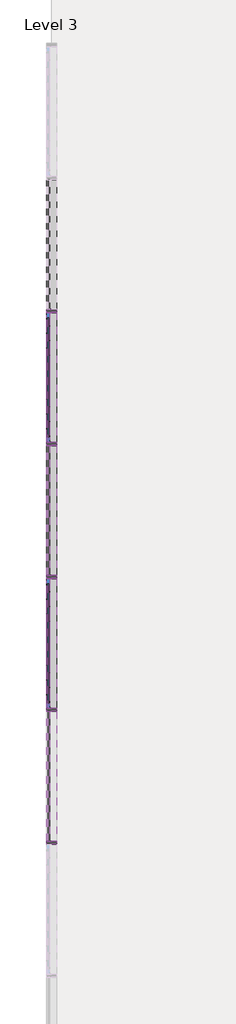
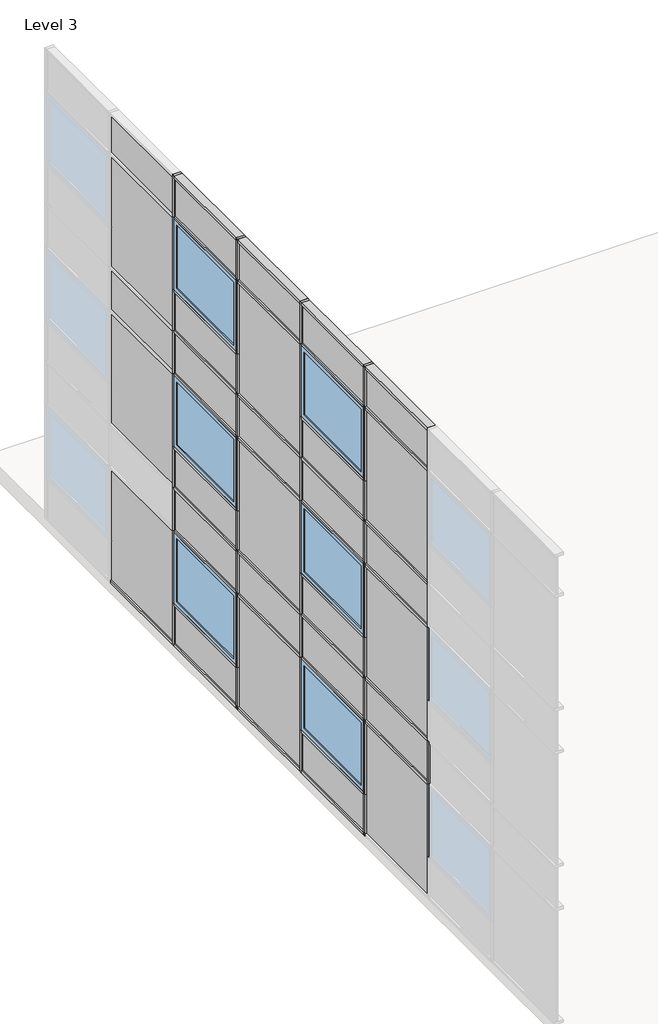
# One storey, part 4 of 5: 73 members, 29 plates, 6 windows.
"""IFC4 building model written with IfcOpenShell, lengths in millimetres."""

import ifcopenshell
import ifcopenshell.guid

model = None  # the IFC model being written
_history = None  # IfcOwnerHistory: only IFC2X3 demands one
_inside = {}  # id of a spatial element -> (the spatial element, [elements in it])
_under = {}  # id of a project, library or spatial element -> (it, [spatial elements below it])
_declared = {}  # id of a project -> (the project, [libraries it declares])
_typed = {}  # id of a type object -> (the type object, [elements of that type])
_made_of = {}  # id of a material, layer set ... -> (it, [elements and type objects made of it])


def new_model(schema):
    """Start an empty IFC model of exactly this schema.

    Asked for "IFC4X3", IfcOpenShell would pick the latest addendum, in which some entities
    have other attributes; the version numbers below select the first issue.
    IFC2X3 requires an IfcOwnerHistory on every rooted entity: one is made here for all.
    """
    global model, _history
    if schema == "IFC4X3":
        model = ifcopenshell.file(schema_version=(4, 3, 0, 0))
    else:
        model = ifcopenshell.file(schema=schema)
    _inside.clear()
    _under.clear()
    _declared.clear()
    _typed.clear()
    _made_of.clear()
    _history = None
    if model.schema == "IFC2X3":
        org = make("IfcOrganization", Name="unknown")
        user = make(
            "IfcPersonAndOrganization",
            ThePerson=make("IfcPerson", FamilyName="unknown"),
            TheOrganization=org,
        )
        app = make(
            "IfcApplication",
            ApplicationDeveloper=org,
            Version="unknown",
            ApplicationFullName="unknown",
            ApplicationIdentifier="unknown",
        )
        _history = make(
            "IfcOwnerHistory",
            OwningUser=user,
            OwningApplication=app,
            ChangeAction="ADDED",
            CreationDate=0,
        )
    return model


def make(cls, **values):
    """One entity of the class cls with the attributes given. An attribute that is None is left unset."""
    return model.create_entity(
        cls, **{name: value for name, value in values.items() if value is not None}
    )


def rooted(cls, **values):
    """An entity with a GlobalId (a new one), such as an element, a storey or a relation."""
    return make(cls, GlobalId=ifcopenshell.guid.new(), OwnerHistory=_history, **values)


def si_unit(unit_type, name, prefix=None):
    """IfcSIUnit, for example si_unit("LENGTHUNIT", "METRE", prefix="MILLI")."""
    return make("IfcSIUnit", UnitType=unit_type, Prefix=prefix, Name=name)


def assignment(units):
    """IfcUnitAssignment: the units of a project."""
    return None if units is None else make("IfcUnitAssignment", Units=units)


def point(xyz):
    """IfcCartesianPoint."""
    return None if xyz is None else make("IfcCartesianPoint", Coordinates=xyz)


def direction(xyz):
    """IfcDirection."""
    return None if xyz is None else make("IfcDirection", DirectionRatios=xyz)


def frame(location, z_axis=None, x_axis=None):
    """IfcAxis2Placement3D, a coordinate frame: its origin and axes. An axis left out is left unset."""
    return make(
        "IfcAxis2Placement3D",
        Location=point(location),
        Axis=direction(z_axis),
        RefDirection=direction(x_axis),
    )


def origin():
    """The frame at (0, 0, 0) with its axes left unset."""
    return frame((0.0, 0.0, 0.0))


def origin_with_axes():
    """The frame at (0, 0, 0) with the z axis (0, 0, 1) and the x axis (1, 0, 0) written out."""
    return frame((0.0, 0.0, 0.0), z_axis=(0.0, 0.0, 1.0), x_axis=(1.0, 0.0, 0.0))


def place(relative_to, where):
    """IfcLocalPlacement: puts the frame where relative to a parent placement (None: the world)."""
    return make(
        "IfcLocalPlacement", PlacementRelTo=relative_to, RelativePlacement=where
    )


def context(
    kind, dimensions, precision=None, world=None, true_north=None, identifier=None
):
    """IfcGeometricRepresentationContext, for example the 3D "Model" context."""
    return make(
        "IfcGeometricRepresentationContext",
        ContextIdentifier=identifier,
        ContextType=kind,
        CoordinateSpaceDimension=dimensions,
        Precision=precision,
        WorldCoordinateSystem=world,
        TrueNorth=true_north,
    )


def project(units=None, contexts=None):
    """IfcProject with its units and contexts."""
    return rooted(
        "IfcProject",
        Name="project",
        RepresentationContexts=contexts,
        UnitsInContext=assignment(units),
    )


def spatial(cls, under=None, at=None, **own):
    """A site, building, storey or space (cls), placed at a placement, below another one or the project."""
    s = rooted(cls, ObjectPlacement=at, **own)
    if under is not None:
        _under.setdefault(under.id(), (under, []))[1].append(s)
    return s


def polyline(points):
    """IfcPolyline through the points."""
    return make("IfcPolyline", Points=[point(p) for p in points])


def outline(outer, holes=None, kind="AREA"):
    """IfcArbitraryClosedProfileDef: a profile drawn as a closed curve; with holes, ...WithVoids."""
    if holes is None:
        return make("IfcArbitraryClosedProfileDef", ProfileType=kind, OuterCurve=outer)
    return make(
        "IfcArbitraryProfileDefWithVoids",
        ProfileType=kind,
        OuterCurve=outer,
        InnerCurves=holes,
    )


def extrude(swept, where, along, depth):
    """IfcExtrudedAreaSolid: the profile swept, set in the frame where, extruded along a direction by depth."""
    return make(
        "IfcExtrudedAreaSolid",
        SweptArea=swept,
        Position=where,
        ExtrudedDirection=direction(along),
        Depth=depth,
    )


def shape(context_of_items, identifier, shape_type, items):
    """IfcShapeRepresentation: the items that make up one representation, for example the "Body"."""
    return make(
        "IfcShapeRepresentation",
        ContextOfItems=context_of_items,
        RepresentationIdentifier=identifier,
        RepresentationType=shape_type,
        Items=items,
    )


def source(mapping_origin, context_of_items, identifier, shape_type, items):
    """IfcRepresentationMap: a shape defined once, which mapped items show again and again."""
    return make(
        "IfcRepresentationMap",
        MappingOrigin=mapping_origin,
        MappedRepresentation=shape(context_of_items, identifier, shape_type, items),
    )


def transform(
    local_origin,
    x_axis=None,
    y_axis=None,
    z_axis=None,
    scale=None,
    scale2=None,
    scale3=None,
    uniform=True,
):
    """IfcCartesianTransformationOperator3D, or its non-uniform kind. x_axis, y_axis, z_axis: its Axis1, 2, 3."""
    if uniform:
        return make(
            "IfcCartesianTransformationOperator3D",
            Axis1=direction(x_axis),
            Axis2=direction(y_axis),
            LocalOrigin=point(local_origin),
            Scale=scale,
            Axis3=direction(z_axis),
        )
    return make(
        "IfcCartesianTransformationOperator3DnonUniform",
        Axis1=direction(x_axis),
        Axis2=direction(y_axis),
        LocalOrigin=point(local_origin),
        Scale=scale,
        Axis3=direction(z_axis),
        Scale2=scale2,
        Scale3=scale3,
    )


def mapped(mapping_source, mapping_target):
    """IfcMappedItem: shows the shape of a source again, moved by a transform."""
    return make(
        "IfcMappedItem", MappingSource=mapping_source, MappingTarget=mapping_target
    )


def made_of(thing, what):
    """Note that an element or type object is made of a material, layer set ...; save() writes the relation."""
    if what is not None:
        _made_of.setdefault(what.id(), (what, []))[1].append(thing)
    return thing


def element(
    cls,
    number,
    at=None,
    inside=None,
    cuts=None,
    type_object=None,
    material=None,
    context=None,
    identifier="Body",
    shape_type=None,
    held_by="IfcProductDefinitionShape",
    body=None,
    shapes=None,
    **own,
):
    """One element of the class cls, such as IfcWall. Its Tag is "e" and its number.

    at: its placement. inside: the storey or other place that contains it. cuts: it is an
    opening in that element (IfcRelVoidsElement). A single representation is given by context,
    identifier, shape_type and body (its items); several are given by shapes. held_by: the class
    of the entity that holds the representations. save() writes the other relations.
    """
    e = rooted(cls, Tag="e%d" % number, ObjectPlacement=at, **own)
    if body is not None:
        shapes = [shape(context, identifier, shape_type, body)]
    if shapes is not None:
        e.Representation = make(held_by, Representations=shapes)
    if inside is not None:
        _inside.setdefault(inside.id(), (inside, []))[1].append(e)
    if cuts is not None:
        rooted(
            "IfcRelVoidsElement", RelatingBuildingElement=cuts, RelatedOpeningElement=e
        )
    if type_object is not None:
        _typed.setdefault(type_object.id(), (type_object, []))[1].append(e)
    return made_of(e, material)


def aggregate(whole, parts):
    """IfcRelAggregates: a whole, such as a stair, and the parts it consists of."""
    return rooted("IfcRelAggregates", RelatingObject=whole, RelatedObjects=parts)


def save(model, path):
    """Write the relations noted so far, then the file.

    IfcRelAggregates (storeys below a building ...), IfcRelContainedInSpatialStructure (elements
    in a storey), IfcRelDefinesByType, IfcRelAssociatesMaterial and IfcRelDeclares: one each for
    every whole, place, type object, material and project.
    """
    for whole, parts in _under.values():
        aggregate(whole, parts)
    for where, things in _inside.values():
        rooted(
            "IfcRelContainedInSpatialStructure",
            RelatedElements=things,
            RelatingStructure=where,
        )
    for kind, things in _typed.values():
        rooted("IfcRelDefinesByType", RelatedObjects=things, RelatingType=kind)
    for what, things in _made_of.values():
        rooted("IfcRelAssociatesMaterial", RelatedObjects=things, RelatingMaterial=what)
    for by, libraries in _declared.values():
        rooted("IfcRelDeclares", RelatingContext=by, RelatedDefinitions=libraries)
    model.write(path)


def rectangular_mullion_50_x_150mm_0967fd3c(model_context):
    return source(origin(), model_context, "Body", "SweptSolid", [
        extrude(outline(polyline([(0.0, 75.0), (0.0, -75.0), (-50.0, -75.0), (-50.0, 75.0), (0.0, 75.0)])), frame((0.0, 0.0, -1950.0000003), z_axis=(0.0, 0.0, 1.0), x_axis=(1.0, 0.0, 0.0)), (0.0, 0.0, 1.0), 1950.0000003),
    ])


def rectangular_mullion_50_x_150mm_f1645b81(model_context):
    return source(origin(), model_context, "Body", "SweptSolid", [
        extrude(outline(polyline([(25.0, 75.0), (25.0, -75.0), (-25.0, -75.0), (-25.0, 75.0), (25.0, 75.0)])), frame((0.0, 0.0, -1950.0000003), z_axis=(0.0, 0.0, 1.0), x_axis=(1.0, 0.0, 0.0)), (0.0, 0.0, 1.0), 1950.0000003),
    ])


def rectangular_mullion_50_x_150mm_14f10ac7(model_context):
    return source(origin(), model_context, "Body", "SweptSolid", [
        extrude(outline(polyline([(25.0, 75.0), (25.0, -75.0), (-25.0, -75.0), (-25.0, 75.0), (25.0, 75.0)])), frame((0.0, 0.0, -800.0), z_axis=(0.0, 0.0, 1.0), x_axis=(1.0, 0.0, 0.0)), (0.0, 0.0, 1.0), 800.0),
    ])


def rectangular_mullion_50_x_150mm_6270d9f9(model_context):
    return source(origin(), model_context, "Body", "SweptSolid", [
        extrude(outline(polyline([(25.0, 75.0), (25.0, -75.0), (-25.0, -75.0), (-25.0, 75.0), (25.0, 75.0)])), frame((0.0, 0.0, -775.0), z_axis=(0.0, 0.0, 1.0), x_axis=(1.0, 0.0, 0.0)), (0.0, 0.0, 1.0), 775.0),
    ])


def rectangular_mullion_50_x_150mm_80d7b263(model_context):
    return source(origin(), model_context, "Body", "SweptSolid", [
        extrude(outline(polyline([(25.0, 75.0), (25.0, -75.0), (-25.0, -75.0), (-25.0, 75.0), (25.0, 75.0)])), frame((0.0, 0.0, -1400.0), z_axis=(0.0, 0.0, 1.0), x_axis=(1.0, 0.0, 0.0)), (0.0, 0.0, 1.0), 1400.0),
    ])


def rectangular_mullion_50_x_150mm_9c26cac3(model_context):
    return source(origin(), model_context, "Body", "SweptSolid", [
        extrude(outline(polyline([(25.0, 75.0), (25.0, -75.0), (-25.0, -75.0), (-25.0, 75.0), (25.0, 75.0)])), frame((0.0, 0.0, -825.0), z_axis=(0.0, 0.0, 1.0), x_axis=(1.0, 0.0, 0.0)), (0.0, 0.0, 1.0), 825.0),
    ])


def system_panel_glazed_1e38db9b(model_context):
    return source(origin(), model_context, "Body", "SweptSolid", [
        extrude(outline(polyline([(0.0, -975.0000002), (0.0, 975.0000002), (750.0, 975.0000002), (2125.0, 975.0000002), (2125.0, -975.0000002), (750.0, -975.0000002), (0.0, -975.0000002)])), frame((0.0, 24.5, 0.0), z_axis=(0.0, 1.0, 0.0), x_axis=(0.0, 0.0, 1.0)), (0.0, 0.0, 1.0), 25.0),
    ])


def system_panel_glazed_bc1ebc0c(model_context):
    return source(origin(), model_context, "Body", "SweptSolid", [
        extrude(outline(polyline([(975.0000002, 24.5), (-975.0000002, 24.5), (-975.0000002, 49.5), (975.0000002, 49.5), (975.0000002, 24.5)])), origin_with_axes(), (0.0, 0.0, 1.0), 725.0),
    ])


def system_panel_glazed_d82c9dbb(model_context):
    return source(origin(), model_context, "Body", "SweptSolid", [
        extrude(outline(polyline([(975.0000002, 24.5), (-975.0000002, 24.5), (-975.0000002, 49.5), (975.0000002, 49.5), (975.0000002, 24.5)])), origin_with_axes(), (0.0, 0.0, 1.0), 775.0),
    ])


def m_curtain_wall_awning_m_curtain_wall_awning_db665c81(model_context):
    return source(origin(), model_context, "Body", "SweptSolid", [
        extrude(outline(polyline([(900.0, 44.05), (-900.0, 44.05), (-900.0, 56.75), (900.0, 56.75), (900.0, 44.05)])), frame((0.0, 0.0, 75.0), z_axis=(0.0, 0.0, 1.0), x_axis=(1.0, 0.0, 0.0)), (0.0, 0.0, 1.0), 1200.0),
        extrude(outline(polyline([(1350.0, -975.0), (0.0, -975.0), (0.0, 975.0), (1350.0, 975.0), (1350.0, -975.0)]), holes=[polyline([(1275.0, -900.0), (1275.0, 900.0), (75.0, 900.0), (75.0, -900.0), (1275.0, -900.0)])]), frame((0.0, 25.0, 0.0), z_axis=(0.0, 1.0, 0.0), x_axis=(0.0, 0.0, 1.0)), (0.0, 0.0, 1.0), 50.0),
    ])


model = new_model("IFC4")

# Units and contexts
model_context = context("Model", 3, world=origin())
ifc_project = project(units=[si_unit("LENGTHUNIT", "METRE", prefix="MILLI")], contexts=[model_context])

# Site, building, storey
site = spatial("IfcSite", under=ifc_project)
building = spatial("IfcBuilding", under=site)
storey = spatial("IfcBuildingStorey", under=building, Name="Level 3", Elevation=6000.0)

# Members
placement = place(None, origin())
rectangular_mullion_50_x_150mm_shape = rectangular_mullion_50_x_150mm_0967fd3c(model_context)
element("IfcMember", 1, ObjectType="Rectangular Mullion : 50 x 150mm", at=placement, inside=storey, context=model_context, shape_type="MappedRepresentation", body=[
    mapped(rectangular_mullion_50_x_150mm_shape, transform((-6732.0028633, 4048.7577233, 6000.0), x_axis=(0.0, 0.0, -1.0), y_axis=(1.0, 0.0, 0.0), z_axis=(0.0, -1.0, 0.0))),
])
element("IfcMember", 2, ObjectType="Rectangular Mullion : 50 x 150mm", at=placement, inside=storey, context=model_context, shape_type="MappedRepresentation", body=[
    mapped(rectangular_mullion_50_x_150mm_shape, transform((-6732.0028633, 6048.7577233, 6000.0), x_axis=(0.0, 0.0, -1.0), y_axis=(1.0, 0.0, 0.0), z_axis=(0.0, -1.0, 0.0))),
])
element("IfcMember", 3, ObjectType="Rectangular Mullion : 50 x 150mm", at=placement, inside=storey, context=model_context, shape_type="MappedRepresentation", body=[
    mapped(rectangular_mullion_50_x_150mm_shape, transform((-6732.0028633, 8048.7577233, 6000.0), x_axis=(0.0, 0.0, -1.0), y_axis=(1.0, 0.0, 0.0), z_axis=(0.0, -1.0, 0.0))),
])
element("IfcMember", 4, ObjectType="Rectangular Mullion : 50 x 150mm", at=placement, inside=storey, context=model_context, shape_type="MappedRepresentation", body=[
    mapped(rectangular_mullion_50_x_150mm_shape, transform((-6732.0028633, 10048.7577233, 6000.0), x_axis=(0.0, 0.0, -1.0), y_axis=(1.0, 0.0, 0.0), z_axis=(0.0, -1.0, 0.0))),
])
rectangular_mullion_50_x_150mm_2_shape = rectangular_mullion_50_x_150mm_f1645b81(model_context)
element("IfcMember", 5, ObjectType="Rectangular Mullion : 50 x 150mm", at=placement, inside=storey, context=model_context, shape_type="MappedRepresentation", body=[
    mapped(rectangular_mullion_50_x_150mm_2_shape, transform((-6732.0028633, 3998.7577233, 14200.0), x_axis=(0.0, 0.0, 1.0), y_axis=(1.0, 0.0, 0.0), z_axis=(0.0, 1.0, 0.0))),
])
element("IfcMember", 6, ObjectType="Rectangular Mullion : 50 x 150mm", at=placement, inside=storey, context=model_context, shape_type="MappedRepresentation", body=[
    mapped(rectangular_mullion_50_x_150mm_2_shape, transform((-6732.0028633, 5998.7577233, 14200.0), x_axis=(0.0, 0.0, 1.0), y_axis=(1.0, 0.0, 0.0), z_axis=(0.0, 1.0, 0.0))),
])
element("IfcMember", 7, ObjectType="Rectangular Mullion : 50 x 150mm", at=placement, inside=storey, context=model_context, shape_type="MappedRepresentation", body=[
    mapped(rectangular_mullion_50_x_150mm_2_shape, transform((-6732.0028633, 7998.7577233, 14200.0), x_axis=(0.0, 0.0, 1.0), y_axis=(1.0, 0.0, 0.0), z_axis=(0.0, 1.0, 0.0))),
])
element("IfcMember", 8, ObjectType="Rectangular Mullion : 50 x 150mm", at=placement, inside=storey, context=model_context, shape_type="MappedRepresentation", body=[
    mapped(rectangular_mullion_50_x_150mm_2_shape, transform((-6732.0028633, 9998.7577233, 14200.0), x_axis=(0.0, 0.0, 1.0), y_axis=(1.0, 0.0, 0.0), z_axis=(0.0, 1.0, 0.0))),
])
element("IfcMember", 9, ObjectType="Rectangular Mullion : 50 x 150mm", at=placement, inside=storey, context=model_context, shape_type="MappedRepresentation", body=[
    mapped(rectangular_mullion_50_x_150mm_2_shape, transform((-6732.0028633, 3998.7577233, 9025.0), x_axis=(0.0, 0.0, 1.0), y_axis=(1.0, 0.0, 0.0), z_axis=(0.0, 1.0, 0.0))),
])
element("IfcMember", 10, ObjectType="Rectangular Mullion : 50 x 150mm", at=placement, inside=storey, context=model_context, shape_type="MappedRepresentation", body=[
    mapped(rectangular_mullion_50_x_150mm_2_shape, transform((-6732.0028633, 5998.7577233, 9025.0), x_axis=(0.0, 0.0, 1.0), y_axis=(1.0, 0.0, 0.0), z_axis=(0.0, 1.0, 0.0))),
])
element("IfcMember", 11, ObjectType="Rectangular Mullion : 50 x 150mm", at=placement, inside=storey, context=model_context, shape_type="MappedRepresentation", body=[
    mapped(rectangular_mullion_50_x_150mm_2_shape, transform((-6732.0028633, 7998.7577233, 9025.0), x_axis=(0.0, 0.0, 1.0), y_axis=(1.0, 0.0, 0.0), z_axis=(0.0, 1.0, 0.0))),
])
element("IfcMember", 12, ObjectType="Rectangular Mullion : 50 x 150mm", at=placement, inside=storey, context=model_context, shape_type="MappedRepresentation", body=[
    mapped(rectangular_mullion_50_x_150mm_2_shape, transform((-6732.0028633, 9998.7577233, 9025.0), x_axis=(0.0, 0.0, 1.0), y_axis=(1.0, 0.0, 0.0), z_axis=(0.0, 1.0, 0.0))),
])
element("IfcMember", 13, ObjectType="Rectangular Mullion : 50 x 150mm", at=placement, inside=storey, context=model_context, shape_type="MappedRepresentation", body=[
    mapped(rectangular_mullion_50_x_150mm_2_shape, transform((-6732.0028633, 3998.7577233, 12025.0), x_axis=(0.0, 0.0, 1.0), y_axis=(1.0, 0.0, 0.0), z_axis=(0.0, 1.0, 0.0))),
])
element("IfcMember", 14, ObjectType="Rectangular Mullion : 50 x 150mm", at=placement, inside=storey, context=model_context, shape_type="MappedRepresentation", body=[
    mapped(rectangular_mullion_50_x_150mm_2_shape, transform((-6732.0028633, 5998.7577233, 12025.0), x_axis=(0.0, 0.0, 1.0), y_axis=(1.0, 0.0, 0.0), z_axis=(0.0, 1.0, 0.0))),
])
element("IfcMember", 15, ObjectType="Rectangular Mullion : 50 x 150mm", at=placement, inside=storey, context=model_context, shape_type="MappedRepresentation", body=[
    mapped(rectangular_mullion_50_x_150mm_2_shape, transform((-6732.0028633, 7998.7577233, 12025.0), x_axis=(0.0, 0.0, 1.0), y_axis=(1.0, 0.0, 0.0), z_axis=(0.0, 1.0, 0.0))),
])
element("IfcMember", 16, ObjectType="Rectangular Mullion : 50 x 150mm", at=placement, inside=storey, context=model_context, shape_type="MappedRepresentation", body=[
    mapped(rectangular_mullion_50_x_150mm_2_shape, transform((-6732.0028633, 9998.7577233, 12025.0), x_axis=(0.0, 0.0, 1.0), y_axis=(1.0, 0.0, 0.0), z_axis=(0.0, 1.0, 0.0))),
])
element("IfcMember", 17, ObjectType="Rectangular Mullion : 50 x 150mm", at=placement, inside=storey, context=model_context, shape_type="MappedRepresentation", body=[
    mapped(rectangular_mullion_50_x_150mm_2_shape, transform((-6732.0028633, 5998.7577233, 12800.0), x_axis=(0.0, 0.0, 1.0), y_axis=(1.0, 0.0, 0.0), z_axis=(0.0, 1.0, 0.0))),
])
element("IfcMember", 18, ObjectType="Rectangular Mullion : 50 x 150mm", at=placement, inside=storey, context=model_context, shape_type="MappedRepresentation", body=[
    mapped(rectangular_mullion_50_x_150mm_2_shape, transform((-6732.0028633, 9998.7577233, 12800.0), x_axis=(0.0, 0.0, 1.0), y_axis=(1.0, 0.0, 0.0), z_axis=(0.0, 1.0, 0.0))),
])
element("IfcMember", 19, ObjectType="Rectangular Mullion : 50 x 150mm", at=placement, inside=storey, context=model_context, shape_type="MappedRepresentation", body=[
    mapped(rectangular_mullion_50_x_150mm_2_shape, transform((-6732.0028633, 3998.7577233, 11200.0), x_axis=(0.0, 0.0, 1.0), y_axis=(1.0, 0.0, 0.0), z_axis=(0.0, 1.0, 0.0))),
])
element("IfcMember", 20, ObjectType="Rectangular Mullion : 50 x 150mm", at=placement, inside=storey, context=model_context, shape_type="MappedRepresentation", body=[
    mapped(rectangular_mullion_50_x_150mm_2_shape, transform((-6732.0028633, 5998.7577233, 11200.0), x_axis=(0.0, 0.0, 1.0), y_axis=(1.0, 0.0, 0.0), z_axis=(0.0, 1.0, 0.0))),
])
element("IfcMember", 21, ObjectType="Rectangular Mullion : 50 x 150mm", at=placement, inside=storey, context=model_context, shape_type="MappedRepresentation", body=[
    mapped(rectangular_mullion_50_x_150mm_2_shape, transform((-6732.0028633, 7998.7577233, 11200.0), x_axis=(0.0, 0.0, 1.0), y_axis=(1.0, 0.0, 0.0), z_axis=(0.0, 1.0, 0.0))),
])
element("IfcMember", 22, ObjectType="Rectangular Mullion : 50 x 150mm", at=placement, inside=storey, context=model_context, shape_type="MappedRepresentation", body=[
    mapped(rectangular_mullion_50_x_150mm_2_shape, transform((-6732.0028633, 9998.7577233, 11200.0), x_axis=(0.0, 0.0, 1.0), y_axis=(1.0, 0.0, 0.0), z_axis=(0.0, 1.0, 0.0))),
])
element("IfcMember", 23, ObjectType="Rectangular Mullion : 50 x 150mm", at=placement, inside=storey, context=model_context, shape_type="MappedRepresentation", body=[
    mapped(rectangular_mullion_50_x_150mm_2_shape, transform((-6732.0028633, 5998.7577233, 9800.0), x_axis=(0.0, 0.0, 1.0), y_axis=(1.0, 0.0, 0.0), z_axis=(0.0, 1.0, 0.0))),
])
element("IfcMember", 24, ObjectType="Rectangular Mullion : 50 x 150mm", at=placement, inside=storey, context=model_context, shape_type="MappedRepresentation", body=[
    mapped(rectangular_mullion_50_x_150mm_2_shape, transform((-6732.0028633, 9998.7577233, 9800.0), x_axis=(0.0, 0.0, 1.0), y_axis=(1.0, 0.0, 0.0), z_axis=(0.0, 1.0, 0.0))),
])
element("IfcMember", 25, ObjectType="Rectangular Mullion : 50 x 150mm", at=placement, inside=storey, context=model_context, shape_type="MappedRepresentation", body=[
    mapped(rectangular_mullion_50_x_150mm_2_shape, transform((-6732.0028633, 3998.7577233, 8200.0), x_axis=(0.0, 0.0, 1.0), y_axis=(1.0, 0.0, 0.0), z_axis=(0.0, 1.0, 0.0))),
])
element("IfcMember", 26, ObjectType="Rectangular Mullion : 50 x 150mm", at=placement, inside=storey, context=model_context, shape_type="MappedRepresentation", body=[
    mapped(rectangular_mullion_50_x_150mm_2_shape, transform((-6732.0028633, 5998.7577233, 8200.0), x_axis=(0.0, 0.0, 1.0), y_axis=(1.0, 0.0, 0.0), z_axis=(0.0, 1.0, 0.0))),
])
element("IfcMember", 27, ObjectType="Rectangular Mullion : 50 x 150mm", at=placement, inside=storey, context=model_context, shape_type="MappedRepresentation", body=[
    mapped(rectangular_mullion_50_x_150mm_2_shape, transform((-6732.0028633, 7998.7577233, 8200.0), x_axis=(0.0, 0.0, 1.0), y_axis=(1.0, 0.0, 0.0), z_axis=(0.0, 1.0, 0.0))),
])
element("IfcMember", 28, ObjectType="Rectangular Mullion : 50 x 150mm", at=placement, inside=storey, context=model_context, shape_type="MappedRepresentation", body=[
    mapped(rectangular_mullion_50_x_150mm_2_shape, transform((-6732.0028633, 9998.7577233, 8200.0), x_axis=(0.0, 0.0, 1.0), y_axis=(1.0, 0.0, 0.0), z_axis=(0.0, 1.0, 0.0))),
])
element("IfcMember", 29, ObjectType="Rectangular Mullion : 50 x 150mm", at=placement, inside=storey, context=model_context, shape_type="MappedRepresentation", body=[
    mapped(rectangular_mullion_50_x_150mm_2_shape, transform((-6732.0028633, 5998.7577233, 6800.0), x_axis=(0.0, 0.0, 1.0), y_axis=(1.0, 0.0, 0.0), z_axis=(0.0, 1.0, 0.0))),
])
element("IfcMember", 30, ObjectType="Rectangular Mullion : 50 x 150mm", at=placement, inside=storey, context=model_context, shape_type="MappedRepresentation", body=[
    mapped(rectangular_mullion_50_x_150mm_2_shape, transform((-6732.0028633, 9998.7577233, 6800.0), x_axis=(0.0, 0.0, 1.0), y_axis=(1.0, 0.0, 0.0), z_axis=(0.0, 1.0, 0.0))),
])
rectangular_mullion_50_x_150mm_3_shape = rectangular_mullion_50_x_150mm_14f10ac7(model_context)
element("IfcMember", 31, ObjectType="Rectangular Mullion : 50 x 150mm", at=placement, inside=storey, context=model_context, shape_type="MappedRepresentation", body=[
    mapped(rectangular_mullion_50_x_150mm_3_shape, transform((-6732.0028633, 4023.7577233, 6000.0), x_axis=(0.0, 1.0, 0.0), y_axis=(1.0, 0.0, 0.0), z_axis=(0.0, 0.0, -1.0))),
])
element("IfcMember", 32, ObjectType="Rectangular Mullion : 50 x 150mm", at=placement, inside=storey, context=model_context, shape_type="MappedRepresentation", body=[
    mapped(rectangular_mullion_50_x_150mm_3_shape, transform((-6732.0028633, 6023.7577233, 6000.0), x_axis=(0.0, 1.0, 0.0), y_axis=(1.0, 0.0, 0.0), z_axis=(0.0, 0.0, -1.0))),
])
element("IfcMember", 33, ObjectType="Rectangular Mullion : 50 x 150mm", at=placement, inside=storey, context=model_context, shape_type="MappedRepresentation", body=[
    mapped(rectangular_mullion_50_x_150mm_3_shape, transform((-6732.0028633, 8023.7577233, 6000.0), x_axis=(0.0, 1.0, 0.0), y_axis=(1.0, 0.0, 0.0), z_axis=(0.0, 0.0, -1.0))),
])
element("IfcMember", 34, ObjectType="Rectangular Mullion : 50 x 150mm", at=placement, inside=storey, context=model_context, shape_type="MappedRepresentation", body=[
    mapped(rectangular_mullion_50_x_150mm_3_shape, transform((-6732.0028633, 10023.7577233, 6000.0), x_axis=(0.0, 1.0, 0.0), y_axis=(1.0, 0.0, 0.0), z_axis=(0.0, 0.0, -1.0))),
])
element("IfcMember", 35, ObjectType="Rectangular Mullion : 50 x 150mm", at=placement, inside=storey, context=model_context, shape_type="MappedRepresentation", body=[
    mapped(rectangular_mullion_50_x_150mm_shape, transform((-6732.0028633, 3998.7577233, 15000.0), x_axis=(0.0, 0.0, 1.0), y_axis=(1.0, 0.0, 0.0), z_axis=(0.0, 1.0, 0.0))),
])
element("IfcMember", 36, ObjectType="Rectangular Mullion : 50 x 150mm", at=placement, inside=storey, context=model_context, shape_type="MappedRepresentation", body=[
    mapped(rectangular_mullion_50_x_150mm_shape, transform((-6732.0028633, 5998.7577233, 15000.0), x_axis=(0.0, 0.0, 1.0), y_axis=(1.0, 0.0, 0.0), z_axis=(0.0, 1.0, 0.0))),
])
element("IfcMember", 37, ObjectType="Rectangular Mullion : 50 x 150mm", at=placement, inside=storey, context=model_context, shape_type="MappedRepresentation", body=[
    mapped(rectangular_mullion_50_x_150mm_shape, transform((-6732.0028633, 7998.7577233, 15000.0), x_axis=(0.0, 0.0, 1.0), y_axis=(1.0, 0.0, 0.0), z_axis=(0.0, 1.0, 0.0))),
])
element("IfcMember", 38, ObjectType="Rectangular Mullion : 50 x 150mm", at=placement, inside=storey, context=model_context, shape_type="MappedRepresentation", body=[
    mapped(rectangular_mullion_50_x_150mm_shape, transform((-6732.0028633, 9998.7577233, 15000.0), x_axis=(0.0, 0.0, 1.0), y_axis=(1.0, 0.0, 0.0), z_axis=(0.0, 1.0, 0.0))),
])
element("IfcMember", 39, ObjectType="Rectangular Mullion : 50 x 150mm", at=placement, inside=storey, context=model_context, shape_type="MappedRepresentation", body=[
    mapped(rectangular_mullion_50_x_150mm_3_shape, transform((-6732.0028633, 4023.7577233, 14200.0), x_axis=(0.0, 1.0, 0.0), y_axis=(1.0, 0.0, 0.0), z_axis=(0.0, 0.0, -1.0))),
])
element("IfcMember", 40, ObjectType="Rectangular Mullion : 50 x 150mm", at=placement, inside=storey, context=model_context, shape_type="MappedRepresentation", body=[
    mapped(rectangular_mullion_50_x_150mm_3_shape, transform((-6732.0028633, 6023.7577233, 14200.0), x_axis=(0.0, 1.0, 0.0), y_axis=(1.0, 0.0, 0.0), z_axis=(0.0, 0.0, -1.0))),
])
element("IfcMember", 41, ObjectType="Rectangular Mullion : 50 x 150mm", at=placement, inside=storey, context=model_context, shape_type="MappedRepresentation", body=[
    mapped(rectangular_mullion_50_x_150mm_3_shape, transform((-6732.0028633, 8023.7577233, 14200.0), x_axis=(0.0, 1.0, 0.0), y_axis=(1.0, 0.0, 0.0), z_axis=(0.0, 0.0, -1.0))),
])
element("IfcMember", 42, ObjectType="Rectangular Mullion : 50 x 150mm", at=placement, inside=storey, context=model_context, shape_type="MappedRepresentation", body=[
    mapped(rectangular_mullion_50_x_150mm_3_shape, transform((-6732.0028633, 10023.7577233, 14200.0), x_axis=(0.0, 1.0, 0.0), y_axis=(1.0, 0.0, 0.0), z_axis=(0.0, 0.0, -1.0))),
])
rectangular_mullion_50_x_150mm_4_shape = rectangular_mullion_50_x_150mm_6270d9f9(model_context)
element("IfcMember", 43, ObjectType="Rectangular Mullion : 50 x 150mm", at=placement, inside=storey, context=model_context, shape_type="MappedRepresentation", body=[
    mapped(rectangular_mullion_50_x_150mm_4_shape, transform((-6732.0028633, 4023.7577233, 9025.0), x_axis=(0.0, 1.0, 0.0), y_axis=(1.0, 0.0, 0.0), z_axis=(0.0, 0.0, -1.0))),
])
element("IfcMember", 44, ObjectType="Rectangular Mullion : 50 x 150mm", at=placement, inside=storey, context=model_context, shape_type="MappedRepresentation", body=[
    mapped(rectangular_mullion_50_x_150mm_4_shape, transform((-6732.0028633, 4023.7577233, 12025.0), x_axis=(0.0, 1.0, 0.0), y_axis=(1.0, 0.0, 0.0), z_axis=(0.0, 0.0, -1.0))),
])
element("IfcMember", 45, ObjectType="Rectangular Mullion : 50 x 150mm", at=placement, inside=storey, context=model_context, shape_type="MappedRepresentation", body=[
    mapped(rectangular_mullion_50_x_150mm_4_shape, transform((-6732.0028633, 6023.7577233, 9025.0), x_axis=(0.0, 1.0, 0.0), y_axis=(1.0, 0.0, 0.0), z_axis=(0.0, 0.0, -1.0))),
])
element("IfcMember", 46, ObjectType="Rectangular Mullion : 50 x 150mm", at=placement, inside=storey, context=model_context, shape_type="MappedRepresentation", body=[
    mapped(rectangular_mullion_50_x_150mm_4_shape, transform((-6732.0028633, 6023.7577233, 12025.0), x_axis=(0.0, 1.0, 0.0), y_axis=(1.0, 0.0, 0.0), z_axis=(0.0, 0.0, -1.0))),
])
element("IfcMember", 47, ObjectType="Rectangular Mullion : 50 x 150mm", at=placement, inside=storey, context=model_context, shape_type="MappedRepresentation", body=[
    mapped(rectangular_mullion_50_x_150mm_4_shape, transform((-6732.0028633, 8023.7577233, 9025.0), x_axis=(0.0, 1.0, 0.0), y_axis=(1.0, 0.0, 0.0), z_axis=(0.0, 0.0, -1.0))),
])
element("IfcMember", 48, ObjectType="Rectangular Mullion : 50 x 150mm", at=placement, inside=storey, context=model_context, shape_type="MappedRepresentation", body=[
    mapped(rectangular_mullion_50_x_150mm_4_shape, transform((-6732.0028633, 8023.7577233, 12025.0), x_axis=(0.0, 1.0, 0.0), y_axis=(1.0, 0.0, 0.0), z_axis=(0.0, 0.0, -1.0))),
])
element("IfcMember", 49, ObjectType="Rectangular Mullion : 50 x 150mm", at=placement, inside=storey, context=model_context, shape_type="MappedRepresentation", body=[
    mapped(rectangular_mullion_50_x_150mm_4_shape, transform((-6732.0028633, 10023.7577233, 9025.0), x_axis=(0.0, 1.0, 0.0), y_axis=(1.0, 0.0, 0.0), z_axis=(0.0, 0.0, -1.0))),
])
element("IfcMember", 50, ObjectType="Rectangular Mullion : 50 x 150mm", at=placement, inside=storey, context=model_context, shape_type="MappedRepresentation", body=[
    mapped(rectangular_mullion_50_x_150mm_4_shape, transform((-6732.0028633, 10023.7577233, 12025.0), x_axis=(0.0, 1.0, 0.0), y_axis=(1.0, 0.0, 0.0), z_axis=(0.0, 0.0, -1.0))),
])
rectangular_mullion_50_x_150mm_5_shape = rectangular_mullion_50_x_150mm_80d7b263(model_context)
element("IfcMember", 51, ObjectType="Rectangular Mullion : 50 x 150mm", at=placement, inside=storey, context=model_context, shape_type="MappedRepresentation", body=[
    mapped(rectangular_mullion_50_x_150mm_5_shape, transform((-6732.0028633, 2023.7577233, 9800.0), x_axis=(0.0, 1.0, 0.0), y_axis=(1.0, 0.0, 0.0), z_axis=(0.0, 0.0, -1.0))),
])
element("IfcMember", 52, ObjectType="Rectangular Mullion : 50 x 150mm", at=placement, inside=storey, context=model_context, shape_type="MappedRepresentation", body=[
    mapped(rectangular_mullion_50_x_150mm_5_shape, transform((-6732.0028633, 2023.7577233, 6800.0), x_axis=(0.0, 1.0, 0.0), y_axis=(1.0, 0.0, 0.0), z_axis=(0.0, 0.0, -1.0))),
])
element("IfcMember", 53, ObjectType="Rectangular Mullion : 50 x 150mm", at=placement, inside=storey, context=model_context, shape_type="MappedRepresentation", body=[
    mapped(rectangular_mullion_50_x_150mm_5_shape, transform((-6732.0028633, 4023.7577233, 12800.0), x_axis=(0.0, 1.0, 0.0), y_axis=(1.0, 0.0, 0.0), z_axis=(0.0, 0.0, -1.0))),
])
element("IfcMember", 54, ObjectType="Rectangular Mullion : 50 x 150mm", at=placement, inside=storey, context=model_context, shape_type="MappedRepresentation", body=[
    mapped(rectangular_mullion_50_x_150mm_5_shape, transform((-6732.0028633, 4023.7577233, 9800.0), x_axis=(0.0, 1.0, 0.0), y_axis=(1.0, 0.0, 0.0), z_axis=(0.0, 0.0, -1.0))),
])
element("IfcMember", 55, ObjectType="Rectangular Mullion : 50 x 150mm", at=placement, inside=storey, context=model_context, shape_type="MappedRepresentation", body=[
    mapped(rectangular_mullion_50_x_150mm_5_shape, transform((-6732.0028633, 4023.7577233, 6800.0), x_axis=(0.0, 1.0, 0.0), y_axis=(1.0, 0.0, 0.0), z_axis=(0.0, 0.0, -1.0))),
])
element("IfcMember", 56, ObjectType="Rectangular Mullion : 50 x 150mm", at=placement, inside=storey, context=model_context, shape_type="MappedRepresentation", body=[
    mapped(rectangular_mullion_50_x_150mm_5_shape, transform((-6732.0028633, 6023.7577233, 12800.0), x_axis=(0.0, 1.0, 0.0), y_axis=(1.0, 0.0, 0.0), z_axis=(0.0, 0.0, -1.0))),
])
element("IfcMember", 57, ObjectType="Rectangular Mullion : 50 x 150mm", at=placement, inside=storey, context=model_context, shape_type="MappedRepresentation", body=[
    mapped(rectangular_mullion_50_x_150mm_5_shape, transform((-6732.0028633, 6023.7577233, 9800.0), x_axis=(0.0, 1.0, 0.0), y_axis=(1.0, 0.0, 0.0), z_axis=(0.0, 0.0, -1.0))),
])
element("IfcMember", 58, ObjectType="Rectangular Mullion : 50 x 150mm", at=placement, inside=storey, context=model_context, shape_type="MappedRepresentation", body=[
    mapped(rectangular_mullion_50_x_150mm_5_shape, transform((-6732.0028633, 6023.7577233, 6800.0), x_axis=(0.0, 1.0, 0.0), y_axis=(1.0, 0.0, 0.0), z_axis=(0.0, 0.0, -1.0))),
])
element("IfcMember", 59, ObjectType="Rectangular Mullion : 50 x 150mm", at=placement, inside=storey, context=model_context, shape_type="MappedRepresentation", body=[
    mapped(rectangular_mullion_50_x_150mm_5_shape, transform((-6732.0028633, 8023.7577233, 12800.0), x_axis=(0.0, 1.0, 0.0), y_axis=(1.0, 0.0, 0.0), z_axis=(0.0, 0.0, -1.0))),
])
element("IfcMember", 60, ObjectType="Rectangular Mullion : 50 x 150mm", at=placement, inside=storey, context=model_context, shape_type="MappedRepresentation", body=[
    mapped(rectangular_mullion_50_x_150mm_5_shape, transform((-6732.0028633, 8023.7577233, 9800.0), x_axis=(0.0, 1.0, 0.0), y_axis=(1.0, 0.0, 0.0), z_axis=(0.0, 0.0, -1.0))),
])
element("IfcMember", 61, ObjectType="Rectangular Mullion : 50 x 150mm", at=placement, inside=storey, context=model_context, shape_type="MappedRepresentation", body=[
    mapped(rectangular_mullion_50_x_150mm_5_shape, transform((-6732.0028633, 8023.7577233, 6800.0), x_axis=(0.0, 1.0, 0.0), y_axis=(1.0, 0.0, 0.0), z_axis=(0.0, 0.0, -1.0))),
])
element("IfcMember", 62, ObjectType="Rectangular Mullion : 50 x 150mm", at=placement, inside=storey, context=model_context, shape_type="MappedRepresentation", body=[
    mapped(rectangular_mullion_50_x_150mm_5_shape, transform((-6732.0028633, 10023.7577233, 12800.0), x_axis=(0.0, 1.0, 0.0), y_axis=(1.0, 0.0, 0.0), z_axis=(0.0, 0.0, -1.0))),
])
element("IfcMember", 63, ObjectType="Rectangular Mullion : 50 x 150mm", at=placement, inside=storey, context=model_context, shape_type="MappedRepresentation", body=[
    mapped(rectangular_mullion_50_x_150mm_5_shape, transform((-6732.0028633, 10023.7577233, 9800.0), x_axis=(0.0, 1.0, 0.0), y_axis=(1.0, 0.0, 0.0), z_axis=(0.0, 0.0, -1.0))),
])
element("IfcMember", 64, ObjectType="Rectangular Mullion : 50 x 150mm", at=placement, inside=storey, context=model_context, shape_type="MappedRepresentation", body=[
    mapped(rectangular_mullion_50_x_150mm_5_shape, transform((-6732.0028633, 10023.7577233, 6800.0), x_axis=(0.0, 1.0, 0.0), y_axis=(1.0, 0.0, 0.0), z_axis=(0.0, 0.0, -1.0))),
])
rectangular_mullion_50_x_150mm_6_shape = rectangular_mullion_50_x_150mm_9c26cac3(model_context)
element("IfcMember", 65, ObjectType="Rectangular Mullion : 50 x 150mm", at=placement, inside=storey, context=model_context, shape_type="MappedRepresentation", body=[
    mapped(rectangular_mullion_50_x_150mm_6_shape, transform((-6732.0028633, 2023.7577233, 8200.0), x_axis=(0.0, 1.0, 0.0), y_axis=(1.0, 0.0, 0.0), z_axis=(0.0, 0.0, -1.0))),
])
element("IfcMember", 66, ObjectType="Rectangular Mullion : 50 x 150mm", at=placement, inside=storey, context=model_context, shape_type="MappedRepresentation", body=[
    mapped(rectangular_mullion_50_x_150mm_6_shape, transform((-6732.0028633, 4023.7577233, 11200.0), x_axis=(0.0, 1.0, 0.0), y_axis=(1.0, 0.0, 0.0), z_axis=(0.0, 0.0, -1.0))),
])
element("IfcMember", 67, ObjectType="Rectangular Mullion : 50 x 150mm", at=placement, inside=storey, context=model_context, shape_type="MappedRepresentation", body=[
    mapped(rectangular_mullion_50_x_150mm_6_shape, transform((-6732.0028633, 4023.7577233, 8200.0), x_axis=(0.0, 1.0, 0.0), y_axis=(1.0, 0.0, 0.0), z_axis=(0.0, 0.0, -1.0))),
])
element("IfcMember", 68, ObjectType="Rectangular Mullion : 50 x 150mm", at=placement, inside=storey, context=model_context, shape_type="MappedRepresentation", body=[
    mapped(rectangular_mullion_50_x_150mm_6_shape, transform((-6732.0028633, 6023.7577233, 11200.0), x_axis=(0.0, 1.0, 0.0), y_axis=(1.0, 0.0, 0.0), z_axis=(0.0, 0.0, -1.0))),
])
element("IfcMember", 69, ObjectType="Rectangular Mullion : 50 x 150mm", at=placement, inside=storey, context=model_context, shape_type="MappedRepresentation", body=[
    mapped(rectangular_mullion_50_x_150mm_6_shape, transform((-6732.0028633, 6023.7577233, 8200.0), x_axis=(0.0, 1.0, 0.0), y_axis=(1.0, 0.0, 0.0), z_axis=(0.0, 0.0, -1.0))),
])
element("IfcMember", 70, ObjectType="Rectangular Mullion : 50 x 150mm", at=placement, inside=storey, context=model_context, shape_type="MappedRepresentation", body=[
    mapped(rectangular_mullion_50_x_150mm_6_shape, transform((-6732.0028633, 8023.7577233, 11200.0), x_axis=(0.0, 1.0, 0.0), y_axis=(1.0, 0.0, 0.0), z_axis=(0.0, 0.0, -1.0))),
])
element("IfcMember", 71, ObjectType="Rectangular Mullion : 50 x 150mm", at=placement, inside=storey, context=model_context, shape_type="MappedRepresentation", body=[
    mapped(rectangular_mullion_50_x_150mm_6_shape, transform((-6732.0028633, 8023.7577233, 8200.0), x_axis=(0.0, 1.0, 0.0), y_axis=(1.0, 0.0, 0.0), z_axis=(0.0, 0.0, -1.0))),
])
element("IfcMember", 72, ObjectType="Rectangular Mullion : 50 x 150mm", at=placement, inside=storey, context=model_context, shape_type="MappedRepresentation", body=[
    mapped(rectangular_mullion_50_x_150mm_6_shape, transform((-6732.0028633, 10023.7577233, 11200.0), x_axis=(0.0, 1.0, 0.0), y_axis=(1.0, 0.0, 0.0), z_axis=(0.0, 0.0, -1.0))),
])
element("IfcMember", 73, ObjectType="Rectangular Mullion : 50 x 150mm", at=placement, inside=storey, context=model_context, shape_type="MappedRepresentation", body=[
    mapped(rectangular_mullion_50_x_150mm_6_shape, transform((-6732.0028633, 10023.7577233, 8200.0), x_axis=(0.0, 1.0, 0.0), y_axis=(1.0, 0.0, 0.0), z_axis=(0.0, 0.0, -1.0))),
])

# Plates
system_panel_glazed_shape = system_panel_glazed_1e38db9b(model_context)
element("IfcPlate", 74, ObjectType="System Panel : Glazed", at=placement, inside=storey, context=model_context, shape_type="MappedRepresentation", body=[
    mapped(system_panel_glazed_shape, transform((-6732.0028633, 3023.7577233, 6050.0), x_axis=(0.0, 1.0, 0.0), y_axis=(-1.0, 0.0, 0.0), z_axis=(0.0, 0.0, 1.0))),
])
element("IfcPlate", 75, ObjectType="System Panel : Glazed", at=placement, inside=storey, context=model_context, shape_type="MappedRepresentation", body=[
    mapped(system_panel_glazed_shape, transform((-6732.0028633, 7023.7577233, 6050.0), x_axis=(0.0, 1.0, 0.0), y_axis=(-1.0, 0.0, 0.0), z_axis=(0.0, 0.0, 1.0))),
])
element("IfcPlate", 76, ObjectType="System Panel : Glazed", at=placement, inside=storey, context=model_context, shape_type="MappedRepresentation", body=[
    mapped(system_panel_glazed_shape, transform((-6732.0028633, 11023.7577233, 6050.0), x_axis=(0.0, 1.0, 0.0), y_axis=(-1.0, 0.0, 0.0), z_axis=(0.0, 0.0, 1.0))),
])
element("IfcPlate", 77, ObjectType="System Panel : Glazed", at=placement, inside=storey, context=model_context, shape_type="MappedRepresentation", body=[
    mapped(system_panel_glazed_shape, transform((-6732.0028633, 3023.7577233, 9050.0), x_axis=(0.0, 1.0, 0.0), y_axis=(-1.0, 0.0, 0.0), z_axis=(0.0, 0.0, 1.0))),
])
element("IfcPlate", 78, ObjectType="System Panel : Glazed", at=placement, inside=storey, context=model_context, shape_type="MappedRepresentation", body=[
    mapped(system_panel_glazed_shape, transform((-6732.0028633, 7023.7577233, 9050.0), x_axis=(0.0, 1.0, 0.0), y_axis=(-1.0, 0.0, 0.0), z_axis=(0.0, 0.0, 1.0))),
])
element("IfcPlate", 79, ObjectType="System Panel : Glazed", at=placement, inside=storey, context=model_context, shape_type="MappedRepresentation", body=[
    mapped(system_panel_glazed_shape, transform((-6732.0028633, 11023.7577233, 9050.0), x_axis=(0.0, 1.0, 0.0), y_axis=(-1.0, 0.0, 0.0), z_axis=(0.0, 0.0, 1.0))),
])
element("IfcPlate", 80, ObjectType="System Panel : Glazed", at=placement, inside=storey, context=model_context, shape_type="MappedRepresentation", body=[
    mapped(system_panel_glazed_shape, transform((-6732.0028633, 3023.7577233, 12050.0), x_axis=(0.0, 1.0, 0.0), y_axis=(-1.0, 0.0, 0.0), z_axis=(0.0, 0.0, 1.0))),
])
element("IfcPlate", 81, ObjectType="System Panel : Glazed", at=placement, inside=storey, context=model_context, shape_type="MappedRepresentation", body=[
    mapped(system_panel_glazed_shape, transform((-6732.0028633, 7023.7577233, 12050.0), x_axis=(0.0, 1.0, 0.0), y_axis=(-1.0, 0.0, 0.0), z_axis=(0.0, 0.0, 1.0))),
])
element("IfcPlate", 82, ObjectType="System Panel : Glazed", at=placement, inside=storey, context=model_context, shape_type="MappedRepresentation", body=[
    mapped(system_panel_glazed_shape, transform((-6732.0028633, 11023.7577233, 12050.0), x_axis=(0.0, 1.0, 0.0), y_axis=(-1.0, 0.0, 0.0), z_axis=(0.0, 0.0, 1.0))),
])
system_panel_glazed_2_shape = system_panel_glazed_bc1ebc0c(model_context)
element("IfcPlate", 83, ObjectType="System Panel : Glazed", at=placement, inside=storey, context=model_context, shape_type="MappedRepresentation", body=[
    mapped(system_panel_glazed_2_shape, transform((-6732.0028633, 3023.7577233, 14225.0), x_axis=(0.0, 1.0, 0.0), y_axis=(-1.0, 0.0, 0.0), z_axis=(0.0, 0.0, 1.0))),
])
element("IfcPlate", 84, ObjectType="System Panel : Glazed", at=placement, inside=storey, context=model_context, shape_type="MappedRepresentation", body=[
    mapped(system_panel_glazed_2_shape, transform((-6732.0028633, 5023.7577233, 6050.0), x_axis=(0.0, 1.0, 0.0), y_axis=(-1.0, 0.0, 0.0), z_axis=(0.0, 0.0, 1.0))),
])
element("IfcPlate", 85, ObjectType="System Panel : Glazed", at=placement, inside=storey, context=model_context, shape_type="MappedRepresentation", body=[
    mapped(system_panel_glazed_2_shape, transform((-6732.0028633, 5023.7577233, 14225.0), x_axis=(0.0, 1.0, 0.0), y_axis=(-1.0, 0.0, 0.0), z_axis=(0.0, 0.0, 1.0))),
])
element("IfcPlate", 86, ObjectType="System Panel : Glazed", at=placement, inside=storey, context=model_context, shape_type="MappedRepresentation", body=[
    mapped(system_panel_glazed_2_shape, transform((-6732.0028633, 7023.7577233, 14225.0), x_axis=(0.0, 1.0, 0.0), y_axis=(-1.0, 0.0, 0.0), z_axis=(0.0, 0.0, 1.0))),
])
element("IfcPlate", 87, ObjectType="System Panel : Glazed", at=placement, inside=storey, context=model_context, shape_type="MappedRepresentation", body=[
    mapped(system_panel_glazed_2_shape, transform((-6732.0028633, 9023.7577233, 6050.0), x_axis=(0.0, 1.0, 0.0), y_axis=(-1.0, 0.0, 0.0), z_axis=(0.0, 0.0, 1.0))),
])
element("IfcPlate", 88, ObjectType="System Panel : Glazed", at=placement, inside=storey, context=model_context, shape_type="MappedRepresentation", body=[
    mapped(system_panel_glazed_2_shape, transform((-6732.0028633, 9023.7577233, 14225.0), x_axis=(0.0, 1.0, 0.0), y_axis=(-1.0, 0.0, 0.0), z_axis=(0.0, 0.0, 1.0))),
])
element("IfcPlate", 89, ObjectType="System Panel : Glazed", at=placement, inside=storey, context=model_context, shape_type="MappedRepresentation", body=[
    mapped(system_panel_glazed_2_shape, transform((-6732.0028633, 11023.7577233, 14225.0), x_axis=(0.0, 1.0, 0.0), y_axis=(-1.0, 0.0, 0.0), z_axis=(0.0, 0.0, 1.0))),
])
element("IfcPlate", 90, ObjectType="System Panel : Glazed", at=placement, inside=storey, context=model_context, shape_type="MappedRepresentation", body=[
    mapped(system_panel_glazed_2_shape, transform((-6732.0028633, 5023.7577233, 9050.0), x_axis=(0.0, 1.0, 0.0), y_axis=(-1.0, 0.0, 0.0), z_axis=(0.0, 0.0, 1.0))),
])
element("IfcPlate", 91, ObjectType="System Panel : Glazed", at=placement, inside=storey, context=model_context, shape_type="MappedRepresentation", body=[
    mapped(system_panel_glazed_2_shape, transform((-6732.0028633, 9023.7577233, 9050.0), x_axis=(0.0, 1.0, 0.0), y_axis=(-1.0, 0.0, 0.0), z_axis=(0.0, 0.0, 1.0))),
])
element("IfcPlate", 92, ObjectType="System Panel : Glazed", at=placement, inside=storey, context=model_context, shape_type="MappedRepresentation", body=[
    mapped(system_panel_glazed_2_shape, transform((-6732.0028633, 5023.7577233, 12050.0), x_axis=(0.0, 1.0, 0.0), y_axis=(-1.0, 0.0, 0.0), z_axis=(0.0, 0.0, 1.0))),
])
element("IfcPlate", 93, ObjectType="System Panel : Glazed", at=placement, inside=storey, context=model_context, shape_type="MappedRepresentation", body=[
    mapped(system_panel_glazed_2_shape, transform((-6732.0028633, 9023.7577233, 12050.0), x_axis=(0.0, 1.0, 0.0), y_axis=(-1.0, 0.0, 0.0), z_axis=(0.0, 0.0, 1.0))),
])
system_panel_glazed_3_shape = system_panel_glazed_d82c9dbb(model_context)
element("IfcPlate", 94, ObjectType="System Panel : Glazed", at=placement, inside=storey, context=model_context, shape_type="MappedRepresentation", body=[
    mapped(system_panel_glazed_3_shape, transform((-6732.0028633, 3023.7577233, 11225.0), x_axis=(0.0, 1.0, 0.0), y_axis=(-1.0, 0.0, 0.0), z_axis=(0.0, 0.0, 1.0))),
])
element("IfcPlate", 95, ObjectType="System Panel : Glazed", at=placement, inside=storey, context=model_context, shape_type="MappedRepresentation", body=[
    mapped(system_panel_glazed_3_shape, transform((-6732.0028633, 5023.7577233, 11225.0), x_axis=(0.0, 1.0, 0.0), y_axis=(-1.0, 0.0, 0.0), z_axis=(0.0, 0.0, 1.0))),
])
element("IfcPlate", 96, ObjectType="System Panel : Glazed", at=placement, inside=storey, context=model_context, shape_type="MappedRepresentation", body=[
    mapped(system_panel_glazed_3_shape, transform((-6732.0028633, 7023.7577233, 11225.0), x_axis=(0.0, 1.0, 0.0), y_axis=(-1.0, 0.0, 0.0), z_axis=(0.0, 0.0, 1.0))),
])
element("IfcPlate", 97, ObjectType="System Panel : Glazed", at=placement, inside=storey, context=model_context, shape_type="MappedRepresentation", body=[
    mapped(system_panel_glazed_3_shape, transform((-6732.0028633, 9023.7577233, 11225.0), x_axis=(0.0, 1.0, 0.0), y_axis=(-1.0, 0.0, 0.0), z_axis=(0.0, 0.0, 1.0))),
])
element("IfcPlate", 98, ObjectType="System Panel : Glazed", at=placement, inside=storey, context=model_context, shape_type="MappedRepresentation", body=[
    mapped(system_panel_glazed_3_shape, transform((-6732.0028633, 11023.7577233, 11225.0), x_axis=(0.0, 1.0, 0.0), y_axis=(-1.0, 0.0, 0.0), z_axis=(0.0, 0.0, 1.0))),
])
element("IfcPlate", 99, ObjectType="System Panel : Glazed", at=placement, inside=storey, context=model_context, shape_type="MappedRepresentation", body=[
    mapped(system_panel_glazed_3_shape, transform((-6732.0028633, 3023.7577233, 8225.0), x_axis=(0.0, 1.0, 0.0), y_axis=(-1.0, 0.0, 0.0), z_axis=(0.0, 0.0, 1.0))),
])
element("IfcPlate", 100, ObjectType="System Panel : Glazed", at=placement, inside=storey, context=model_context, shape_type="MappedRepresentation", body=[
    mapped(system_panel_glazed_3_shape, transform((-6732.0028633, 5023.7577233, 8225.0), x_axis=(0.0, 1.0, 0.0), y_axis=(-1.0, 0.0, 0.0), z_axis=(0.0, 0.0, 1.0))),
])
element("IfcPlate", 101, ObjectType="System Panel : Glazed", at=placement, inside=storey, context=model_context, shape_type="MappedRepresentation", body=[
    mapped(system_panel_glazed_3_shape, transform((-6732.0028633, 7023.7577233, 8225.0), x_axis=(0.0, 1.0, 0.0), y_axis=(-1.0, 0.0, 0.0), z_axis=(0.0, 0.0, 1.0))),
])
element("IfcPlate", 102, ObjectType="System Panel : Glazed", at=placement, inside=storey, context=model_context, shape_type="MappedRepresentation", body=[
    mapped(system_panel_glazed_3_shape, transform((-6732.0028633, 9023.7577233, 8225.0), x_axis=(0.0, 1.0, 0.0), y_axis=(-1.0, 0.0, 0.0), z_axis=(0.0, 0.0, 1.0))),
])

# Windows
m_curtain_wall_awning_m_curtain_wall_awning_shape = m_curtain_wall_awning_m_curtain_wall_awning_db665c81(model_context)
element("IfcWindow", 103, ObjectType="M_Curtain Wall Awning : M_Curtain Wall Awning", at=placement, inside=storey, context=model_context, shape_type="MappedRepresentation", body=[
    mapped(m_curtain_wall_awning_m_curtain_wall_awning_shape, transform((-6732.0028633, 5023.7577233, 12825.0), x_axis=(0.0, 1.0, 0.0), y_axis=(-1.0, 0.0, 0.0), z_axis=(0.0, 0.0, 1.0))),
])
element("IfcWindow", 104, ObjectType="M_Curtain Wall Awning : M_Curtain Wall Awning", at=placement, inside=storey, context=model_context, shape_type="MappedRepresentation", body=[
    mapped(m_curtain_wall_awning_m_curtain_wall_awning_shape, transform((-6732.0028633, 9023.7577233, 12825.0), x_axis=(0.0, 1.0, 0.0), y_axis=(-1.0, 0.0, 0.0), z_axis=(0.0, 0.0, 1.0))),
])
element("IfcWindow", 105, ObjectType="M_Curtain Wall Awning : M_Curtain Wall Awning", at=placement, inside=storey, context=model_context, shape_type="MappedRepresentation", body=[
    mapped(m_curtain_wall_awning_m_curtain_wall_awning_shape, transform((-6732.0028633, 5023.7577233, 9825.0), x_axis=(0.0, 1.0, 0.0), y_axis=(-1.0, 0.0, 0.0), z_axis=(0.0, 0.0, 1.0))),
])
element("IfcWindow", 106, ObjectType="M_Curtain Wall Awning : M_Curtain Wall Awning", at=placement, inside=storey, context=model_context, shape_type="MappedRepresentation", body=[
    mapped(m_curtain_wall_awning_m_curtain_wall_awning_shape, transform((-6732.0028633, 9023.7577233, 9825.0), x_axis=(0.0, 1.0, 0.0), y_axis=(-1.0, 0.0, 0.0), z_axis=(0.0, 0.0, 1.0))),
])
element("IfcWindow", 107, ObjectType="M_Curtain Wall Awning : M_Curtain Wall Awning", at=placement, inside=storey, context=model_context, shape_type="MappedRepresentation", body=[
    mapped(m_curtain_wall_awning_m_curtain_wall_awning_shape, transform((-6732.0028633, 5023.7577233, 6825.0), x_axis=(0.0, 1.0, 0.0), y_axis=(-1.0, 0.0, 0.0), z_axis=(0.0, 0.0, 1.0))),
])
element("IfcWindow", 108, ObjectType="M_Curtain Wall Awning : M_Curtain Wall Awning", at=placement, inside=storey, context=model_context, shape_type="MappedRepresentation", body=[
    mapped(m_curtain_wall_awning_m_curtain_wall_awning_shape, transform((-6732.0028633, 9023.7577233, 6825.0), x_axis=(0.0, 1.0, 0.0), y_axis=(-1.0, 0.0, 0.0), z_axis=(0.0, 0.0, 1.0))),
])

save(model, "model.ifc")

# Revit data of these elements
# Type "Rectangular Mullion : 50 x 150mm"
#   built-in parameter 1007304 = 0.492126 (stored number, unit not read)
#   built-in parameter 1007301 = 0.082021 (stored number, unit not read)
#   built-in parameter 1007300 = 0.082021 (stored number, unit not read)
# Type "M_Curtain Wall Awning : M_Curtain Wall Awning"
#   Type Mark = "20"
#   Offset = 0.075 m
#   Sash Width = 0.075 m
#   Thickness = 0.050 m
#   Define Thermal Properties by = 1
#   Glass Pane Material = Window - Glass
#   Sash Material = Metal - Aluminum
# Elements 1, 2, 3, 4, 5, 6, 7, 8, 9, 10, 11, 12, 13, 14, 15, 16, 17, 18, 19, 20, 21, 22, 23, 24, 25, 26, 27, 28, 29, 30, 31, 32, 33, 34, 35, 36, 37, 38, 39, 40, 41, 42, 43, 44, 45, 46, 47, 48, 49, 50, 51, 52, 53, 54, 55, 56, 57, 58, 59, 60, 61, 62, 63, 64, 65, 66, 67, 68, 69, 70, 71, 72, 73 (IfcMember, "Rectangular Mullion : 50 x 150mm")
#   Phase Created = New Construction
#   Materials on its faces: "Metal - Aluminium"
# Elements 74, 75, 76, 77, 78, 79, 80, 81, 82, 83, 84, 85, 86, 87, 88, 89, 90, 91, 92, 93, 94, 95, 96, 97, 98, 99, 100, 101, 102 (IfcPlate, "System Panel : Glazed")
#   Phase Created = New Construction
#   Materials on its faces: "Glass"
# Elements 103, 104, 105, 106, 107, 108 (IfcWindow, "M_Curtain Wall Awning : M_Curtain Wall Awning")
#   Phase Created = New Construction
#   Materials on its faces: "Metal - Aluminum", "Window - Glass"
# Materials
#   "Window - Glass": class "Glas", colour RGB 128 128 255, transparency 0.75
#   "Metal - Aluminum": class "Unassigned", colour RGB 247 247 247, transparency 0, Comments = "Rendering appearance not upgraded "
#   "Metal - Aluminium": class "Metal", colour RGB 247 247 247, transparency 0
#   "Glass": class "Glass", colour RGB 0 128 192, transparency 0.9
